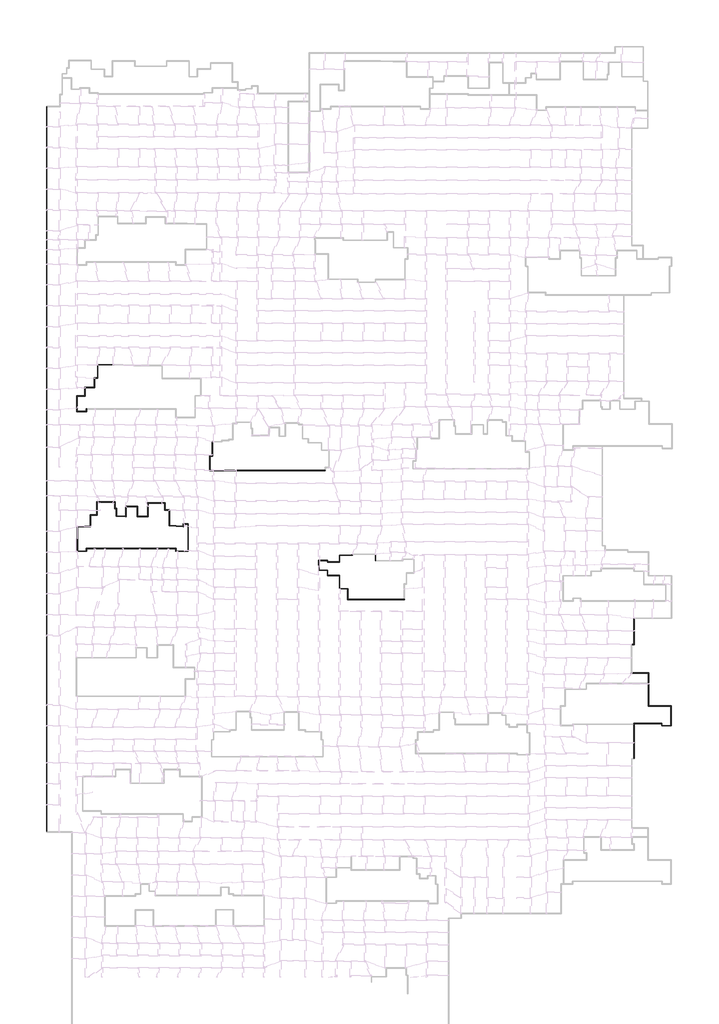
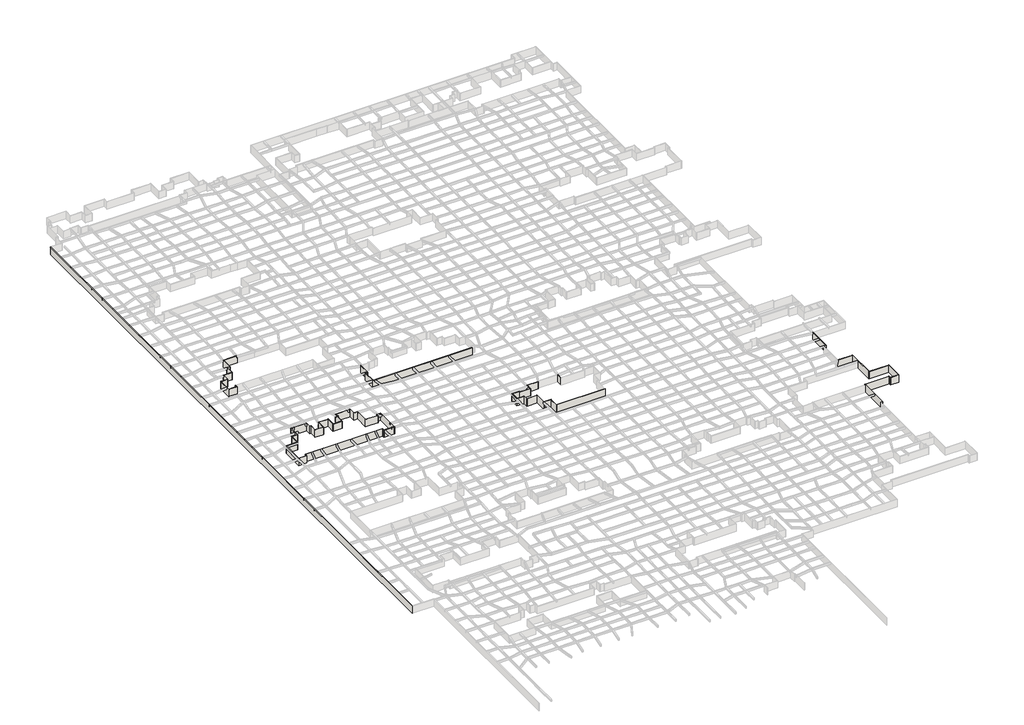
# One storey, part 5 of 45: 68 walls.
"""IFC4 building model written with IfcOpenShell, lengths in millimetres."""

from ifc_helpers import new_model, si_unit, origin, origin_with_axes, place, context, project, spatial, polyline, outline, extrude, faceted_brep, element, save

model = new_model("IFC4")

# Units and contexts
model_context = context("Model", 3, world=origin())
ifc_project = project(units=[si_unit("LENGTHUNIT", "METRE", prefix="MILLI")], contexts=[model_context])

# Site, building, storey
site = spatial("IfcSite", under=ifc_project)
building = spatial("IfcBuilding", under=site)
storey = spatial("IfcBuildingStorey", under=building, Name="户型图", Elevation=0.0)

# Walls
placement = place(None, origin())
element("IfcWall", 1, ObjectType="所有墙体", at=placement, inside=storey, context=model_context, shape_type="Brep", body=[
    faceted_brep([(-155100.5216564, 191211.9876735, 0.0), (-155100.5216564, -79588.0123265, 0.0), (-155100.5216564, -79588.0123265, 3300.0), (-155100.5216564, 191211.9876735, 3300.0), (-154980.5216564, 191211.9876735, 0.0), (-154980.5216564, 191211.9876735, 3300.0), (-154980.5216564, -79468.0123265, 3300.0), (-154980.5216564, -79588.0123265, 3300.0), (-154980.5216564, -79588.0123265, 0.0), (-154980.5216564, -79468.0123265, 0.0)], [[[0, 1, 2, 3]], [[4, 5, 6, 7, 8, 9]], [[1, 0, 4, 9, 8]], [[3, 2, 7, 6, 5]], [[0, 3, 5, 4]], [[2, 1, 8, 7]]]),
])
element("IfcWall", 2, ObjectType="所有墙体", at=placement, inside=storey, context=model_context, shape_type="Brep", body=[
    faceted_brep([(64319.4783436, -52068.0123265, 0.0), (64319.4783436, -38988.0123265, 0.0), (64319.4783436, -38868.0123265, 0.0), (64319.4783436, -38868.0123265, 3300.0), (64319.4783436, -38988.0123265, 3300.0), (64319.4783436, -52068.0123265, 3300.0), (64199.4783436, -52068.0123265, 0.0), (64199.4783436, -52068.0123265, 3300.0), (64199.4783436, -39338.8304418, 3300.0), (64199.4783436, -39218.8304418, 3300.0), (64199.4783436, -38868.0123265, 3300.0), (64199.4783436, -38868.0123265, 0.0), (64199.4783436, -39218.8304418, 0.0), (64199.4783436, -39338.8304418, 0.0)], [[[0, 1, 2, 3, 4, 5]], [[6, 7, 8, 9, 10, 11, 12, 13]], [[2, 1, 0, 6, 13, 12, 11]], [[5, 4, 3, 10, 9, 8, 7]], [[0, 5, 7, 6]], [[3, 2, 11, 10]]]),
])
element("IfcWall", 3, ObjectType="所有墙体", at=placement, inside=storey, context=model_context, shape_type="Brep", body=[
    faceted_brep([(64319.4783436, -38988.0123265, 0.0), (74599.4783436, -38988.0123265, 0.0), (74719.4783436, -38988.0123265, 0.0), (74719.4783436, -38988.0123265, 3300.0), (74599.4783436, -38988.0123265, 3300.0), (64319.4783436, -38988.0123265, 3300.0), (64319.4783436, -38868.0123265, 0.0), (64319.4783436, -38868.0123265, 3300.0), (74719.4783436, -38868.0123265, 3300.0), (74719.4783436, -38868.0123265, 0.0)], [[[0, 1, 2, 3, 4, 5]], [[6, 7, 8, 9]], [[2, 1, 0, 6, 9]], [[5, 4, 3, 8, 7]], [[0, 5, 7, 6]], [[3, 2, 9, 8]]]),
])
element("IfcWall", 4, ObjectType="所有墙体", at=placement, inside=storey, context=model_context, shape_type="Brep", body=[
    faceted_brep([(74599.4783436, -38988.0123265, 0.0), (74599.4783436, -39888.0123265, 0.0), (74599.4783436, -39888.0123265, 3300.0), (74599.4783436, -38988.0123265, 3300.0), (74719.4783436, -38988.0123265, 0.0), (74719.4783436, -38988.0123265, 3300.0), (74719.4783436, -39768.0123265, 3300.0), (74719.4783436, -39888.0123265, 3300.0), (74719.4783436, -39888.0123265, 0.0), (74719.4783436, -39768.0123265, 0.0)], [[[0, 1, 2, 3]], [[4, 5, 6, 7, 8, 9]], [[1, 0, 4, 9, 8]], [[3, 2, 7, 6, 5]], [[0, 3, 5, 4]], [[2, 1, 8, 7]]]),
])
element("IfcWall", 5, ObjectType="所有墙体", at=placement, inside=storey, context=model_context, shape_type="Brep", body=[
    faceted_brep([(74719.4783436, -39888.0123265, 0.0), (78219.4783436, -39888.0123265, 0.0), (78219.4783436, -39888.0123265, 3300.0), (74719.4783436, -39888.0123265, 3300.0), (74719.4783436, -39768.0123265, 0.0), (74719.4783436, -39768.0123265, 3300.0), (78099.4783436, -39768.0123265, 3300.0), (78219.4783436, -39768.0123265, 3300.0), (78219.4783436, -39768.0123265, 0.0), (78099.4783436, -39768.0123265, 0.0)], [[[0, 1, 2, 3]], [[4, 5, 6, 7, 8, 9]], [[1, 0, 4, 9, 8]], [[3, 2, 7, 6, 5]], [[0, 3, 5, 4]], [[2, 1, 8, 7]]]),
])
element("IfcWall", 6, ObjectType="所有墙体", at=placement, inside=storey, context=model_context, shape_type="Brep", body=[
    faceted_brep([(78219.4783436, -39768.0123265, 0.0), (78219.4783436, -32368.0123265, 0.0), (78219.4783436, -32368.0123265, 3300.0), (78219.4783436, -39768.0123265, 3300.0), (78099.4783436, -39768.0123265, 0.0), (78099.4783436, -39768.0123265, 3300.0), (78099.4783436, -32488.0123265, 3300.0), (78099.4783436, -32368.0123265, 3300.0), (78099.4783436, -32368.0123265, 0.0), (78099.4783436, -32488.0123265, 0.0)], [[[0, 1, 2, 3]], [[4, 5, 6, 7, 8, 9]], [[1, 0, 4, 9, 8]], [[3, 2, 7, 6, 5]], [[0, 3, 5, 4]], [[2, 1, 8, 7]]]),
])
element("IfcWall", 7, ObjectType="所有墙体", at=placement, inside=storey, context=model_context, shape_type="Brep", body=[
    faceted_brep([(78099.4783436, -32368.0123265, 0.0), (69819.4783436, -32368.0123265, 0.0), (69699.4783436, -32368.0123265, 0.0), (69699.4783436, -32368.0123265, 3300.0), (69819.4783436, -32368.0123265, 3300.0), (78099.4783436, -32368.0123265, 3300.0), (78099.4783436, -32488.0123265, 0.0), (78099.4783436, -32488.0123265, 3300.0), (69699.4783436, -32488.0123265, 3300.0), (69699.4783436, -32488.0123265, 0.0)], [[[0, 1, 2, 3, 4, 5]], [[6, 7, 8, 9]], [[2, 1, 0, 6, 9]], [[5, 4, 3, 8, 7]], [[0, 5, 7, 6]], [[3, 2, 9, 8]]]),
])
element("IfcWall", 8, ObjectType="所有墙体", at=placement, inside=storey, context=model_context, shape_type="Brep", body=[
    faceted_brep([(69819.4783436, -32368.0123265, 0.0), (69819.4783436, -20068.0123265, 0.0), (69819.4783436, -20068.0123265, 3300.0), (69819.4783436, -32368.0123265, 3300.0), (69699.4783436, -32368.0123265, 0.0), (69699.4783436, -32368.0123265, 3300.0), (69699.4783436, -24130.6851163, 3300.0), (69699.4783436, -24010.6851163, 3300.0), (69699.4783436, -20188.0123265, 3300.0), (69699.4783436, -20068.0123265, 3300.0), (69699.4783436, -20068.0123265, 0.0), (69699.4783436, -20188.0123265, 0.0), (69699.4783436, -24010.6851163, 0.0), (69699.4783436, -24130.6851163, 0.0)], [[[0, 1, 2, 3]], [[4, 5, 6, 7, 8, 9, 10, 11, 12, 13]], [[1, 0, 4, 13, 12, 11, 10]], [[3, 2, 9, 8, 7, 6, 5]], [[0, 3, 5, 4]], [[2, 1, 10, 9]]]),
])
element("IfcWall", 9, ObjectType="所有墙体", at=placement, inside=storey, context=model_context, shape_type="Brep", body=[
    faceted_brep([(69699.4783436, -20068.0123265, 0.0), (63419.4783436, -20068.0123265, 0.0), (63299.4783436, -20068.0123265, 0.0), (63299.4783436, -20068.0123265, 3300.0), (63419.4783436, -20068.0123265, 3300.0), (69699.4783436, -20068.0123265, 3300.0), (69699.4783436, -20188.0123265, 0.0), (69699.4783436, -20188.0123265, 3300.0), (63299.4783436, -20188.0123265, 3300.0), (63299.4783436, -20188.0123265, 0.0)], [[[0, 1, 2, 3, 4, 5]], [[6, 7, 8, 9]], [[2, 1, 0, 6, 9]], [[5, 4, 3, 8, 7]], [[0, 5, 7, 6]], [[3, 2, 9, 8]]]),
])
element("IfcWall", 10, ObjectType="所有墙体", at=placement, inside=storey, context=model_context, shape_type="Brep", body=[
    faceted_brep([(63419.4783436, -9588.0123265, 0.0), (64419.4783436, -9588.0123265, 0.0), (64419.4783436, -9588.0123265, 3300.0), (63419.4783436, -9588.0123265, 3300.0), (63419.4783436, -9468.0123265, 0.0), (63419.4783436, -9468.0123265, 3300.0), (64299.4783436, -9468.0123265, 3300.0), (64419.4783436, -9468.0123265, 3300.0), (64419.4783436, -9468.0123265, 0.0), (64299.4783436, -9468.0123265, 0.0)], [[[0, 1, 2, 3]], [[4, 5, 6, 7, 8, 9]], [[1, 0, 4, 9, 8]], [[3, 2, 7, 6, 5]], [[0, 3, 5, 4]], [[2, 1, 8, 7]]]),
])
element("IfcWall", 11, ObjectType="所有墙体", at=placement, inside=storey, context=model_context, shape_type="Brep", body=[
    faceted_brep([(64419.4783436, -9468.0123265, 0.0), (64419.4783436, 211.9876735, 0.0), (64419.4783436, 331.9876735, 0.0), (64419.4783436, 331.9876735, 3300.0), (64419.4783436, 211.9876735, 3300.0), (64419.4783436, -9468.0123265, 3300.0), (64299.4783436, -9468.0123265, 0.0), (64299.4783436, -9468.0123265, 3300.0), (64299.4783436, 331.9876735, 3300.0), (64299.4783436, 331.9876735, 0.0)], [[[0, 1, 2, 3, 4, 5]], [[6, 7, 8, 9]], [[2, 1, 0, 6, 9]], [[5, 4, 3, 8, 7]], [[0, 5, 7, 6]], [[3, 2, 9, 8]]]),
])
element("IfcWall", 12, ObjectType="所有墙体", at=placement, inside=storey, context=model_context, shape_type="Brep", body=[
    faceted_brep([(-136051.3875586, 94934.6670053, 0.0), (-136051.3875586, 90014.2865852, 0.0), (-136051.3875586, 89894.2865852, 0.0), (-136051.3875586, 89894.2865852, 3300.0), (-136051.3875586, 90014.2865852, 3300.0), (-136051.3875586, 94934.6670053, 3300.0), (-135931.3875586, 94934.6670053, 0.0), (-135931.3875586, 94934.6670053, 3300.0), (-135931.3875586, 94814.6670053, 3300.0), (-135931.3875586, 89894.2865852, 3300.0), (-135931.3875586, 89894.2865852, 0.0), (-135931.3875586, 94814.6670053, 0.0)], [[[0, 1, 2, 3, 4, 5]], [[6, 7, 8, 9, 10, 11]], [[2, 1, 0, 6, 11, 10]], [[5, 4, 3, 9, 8, 7]], [[3, 2, 10, 9]], [[0, 5, 7, 6]]]),
])
element("IfcWall", 13, ObjectType="所有墙体", at=placement, inside=storey, context=model_context, shape_type="Brep", body=[
    faceted_brep([(-136051.3875586, 90014.2865852, 0.0), (-137251.3875586, 90014.2865852, 0.0), (-137251.3875586, 90014.2865852, 3300.0), (-136051.3875586, 90014.2865852, 3300.0), (-136051.3875586, 89894.2865852, 0.0), (-136051.3875586, 89894.2865852, 3300.0), (-137131.3875586, 89894.2865852, 3300.0), (-137251.3875586, 89894.2865852, 3300.0), (-137251.3875586, 89894.2865852, 0.0), (-137131.3875586, 89894.2865852, 0.0)], [[[0, 1, 2, 3]], [[4, 5, 6, 7, 8, 9]], [[1, 0, 4, 9, 8]], [[3, 2, 7, 6, 5]], [[0, 3, 5, 4]], [[2, 1, 8, 7]]]),
])
element("IfcWall", 14, ObjectType="所有墙体", at=placement, inside=storey, context=model_context, shape_type="Brep", body=[
    faceted_brep([(-137251.3875586, 89894.2865852, 0.0), (-137251.3875586, 86414.2865852, 0.0), (-137251.3875586, 86294.2865852, 0.0), (-137251.3875586, 86294.2865852, 3300.0), (-137251.3875586, 86414.2865852, 3300.0), (-137251.3875586, 89894.2865852, 3300.0), (-137131.3875586, 89894.2865852, 0.0), (-137131.3875586, 89894.2865852, 3300.0), (-137131.3875586, 86294.2865852, 3300.0), (-137131.3875586, 86294.2865852, 0.0)], [[[0, 1, 2, 3, 4, 5]], [[6, 7, 8, 9]], [[2, 1, 0, 6, 9]], [[5, 4, 3, 8, 7]], [[0, 5, 7, 6]], [[3, 2, 9, 8]]]),
])
element("IfcWall", 15, ObjectType="所有墙体", at=placement, inside=storey, context=model_context, shape_type="Brep", body=[
    faceted_brep([(-137251.3875586, 86414.2865852, 0.0), (-140851.3875586, 86414.2865852, 0.0), (-140851.3875586, 86414.2865852, 3300.0), (-137251.3875586, 86414.2865852, 3300.0), (-137251.3875586, 86294.2865852, 0.0), (-137251.3875586, 86294.2865852, 3300.0), (-140731.3875586, 86294.2865852, 3300.0), (-140851.3875586, 86294.2865852, 3300.0), (-140851.3875586, 86294.2865852, 0.0), (-140731.3875586, 86294.2865852, 0.0)], [[[0, 1, 2, 3]], [[4, 5, 6, 7, 8, 9]], [[1, 0, 4, 9, 8]], [[3, 2, 7, 6, 5]], [[0, 3, 5, 4]], [[2, 1, 8, 7]]]),
])
element("IfcWall", 16, ObjectType="所有墙体", at=placement, inside=storey, context=model_context, shape_type="Brep", body=[
    faceted_brep([(-140851.3875586, 86294.2865852, 0.0), (-140851.3875586, 83314.2865852, 0.0), (-140851.3875586, 83194.2865852, 0.0), (-140851.3875586, 83194.2865852, 3300.0), (-140851.3875586, 83314.2865852, 3300.0), (-140851.3875586, 86294.2865852, 3300.0), (-140731.3875586, 86294.2865852, 0.0), (-140731.3875586, 86294.2865852, 3300.0), (-140731.3875586, 83194.2865852, 3300.0), (-140731.3875586, 83194.2865852, 0.0)], [[[0, 1, 2, 3, 4, 5]], [[6, 7, 8, 9]], [[2, 1, 0, 6, 9]], [[5, 4, 3, 8, 7]], [[0, 5, 7, 6]], [[3, 2, 9, 8]]]),
])
element("IfcWall", 17, ObjectType="所有墙体", at=placement, inside=storey, context=model_context, shape_type="Brep", body=[
    faceted_brep([(-140851.3875586, 83314.2865852, 0.0), (-143751.3875586, 83314.2865852, 0.0), (-143751.3875586, 83314.2865852, 3300.0), (-140851.3875586, 83314.2865852, 3300.0), (-140851.3875586, 83194.2865852, 0.0), (-140851.3875586, 83194.2865852, 3300.0), (-143631.3875586, 83194.2865852, 3300.0), (-143751.3875586, 83194.2865852, 3300.0), (-143751.3875586, 83194.2865852, 0.0), (-143631.3875586, 83194.2865852, 0.0)], [[[0, 1, 2, 3]], [[4, 5, 6, 7, 8, 9]], [[1, 0, 4, 9, 8]], [[3, 2, 7, 6, 5]], [[0, 3, 5, 4]], [[2, 1, 8, 7]]]),
])
element("IfcWall", 18, ObjectType="所有墙体", at=placement, inside=storey, context=model_context, shape_type="Brep", body=[
    faceted_brep([(-143751.3875586, 83194.2865852, 0.0), (-143751.3875586, 77394.2865852, 0.0), (-143751.3875586, 77394.2865852, 3300.0), (-143751.3875586, 83194.2865852, 3300.0), (-143631.3875586, 83194.2865852, 0.0), (-143631.3875586, 83194.2865852, 3300.0), (-143631.3875586, 77514.2865852, 3300.0), (-143631.3875586, 77394.2865852, 3300.0), (-143631.3875586, 77394.2865852, 0.0), (-143631.3875586, 77514.2865852, 0.0)], [[[0, 1, 2, 3]], [[4, 5, 6, 7, 8, 9]], [[1, 0, 4, 9, 8]], [[3, 2, 7, 6, 5]], [[0, 3, 5, 4]], [[2, 1, 8, 7]]]),
])
element("IfcWall", 19, ObjectType="所有墙体", at=placement, inside=storey, context=model_context, shape_type="Brep", body=[
    faceted_brep([(-143631.3875586, 77394.2865852, 0.0), (-140131.3875586, 77394.2865852, 0.0), (-140131.3875586, 77394.2865852, 3300.0), (-143631.3875586, 77394.2865852, 3300.0), (-143631.3875586, 77514.2865852, 0.0), (-143631.3875586, 77514.2865852, 3300.0), (-140251.3875586, 77514.2865852, 3300.0), (-140131.3875586, 77514.2865852, 3300.0), (-140131.3875586, 77514.2865852, 0.0), (-140251.3875586, 77514.2865852, 0.0)], [[[0, 1, 2, 3]], [[4, 5, 6, 7, 8, 9]], [[1, 0, 4, 9, 8]], [[3, 2, 7, 6, 5]], [[0, 3, 5, 4]], [[2, 1, 8, 7]]]),
])
element("IfcWall", 20, ObjectType="所有墙体", at=placement, inside=storey, context=model_context, shape_type="Brep", body=[
    faceted_brep([(-140131.3875586, 77514.2865852, 0.0), (-140131.3875586, 78294.2865852, 0.0), (-140131.3875586, 78414.2865852, 0.0), (-140131.3875586, 78414.2865852, 3300.0), (-140131.3875586, 78294.2865852, 3300.0), (-140131.3875586, 77514.2865852, 3300.0), (-140251.3875586, 77514.2865852, 0.0), (-140251.3875586, 77514.2865852, 3300.0), (-140251.3875586, 78414.2865852, 3300.0), (-140251.3875586, 78414.2865852, 0.0)], [[[0, 1, 2, 3, 4, 5]], [[6, 7, 8, 9]], [[2, 1, 0, 6, 9]], [[5, 4, 3, 8, 7]], [[0, 5, 7, 6]], [[3, 2, 9, 8]]]),
])
element("IfcWall", 21, ObjectType="所有墙体", at=placement, inside=storey, context=model_context, shape_type="SweptSolid", body=[
    extrude(outline(polyline([(-135931.3875586, 94934.6670053), (-129985.7714573, 94934.6670053), (-129987.8660651, 94814.6670053), (-135931.3875586, 94814.6670053), (-135931.3875586, 94934.6670053)])), origin_with_axes(), (0.0, 0.0, 1.0), 3300.0),
])
element("IfcWall", 22, ObjectType="所有墙体", at=placement, inside=storey, context=model_context, shape_type="Brep", body=[
    faceted_brep([(-51113.897353, 55455.9851813, 0.0), (-93993.897353, 55455.9851813, 0.0), (-94113.897353, 55455.9851813, 0.0), (-94113.897353, 55455.9851813, 3300.0), (-93993.897353, 55455.9851813, 3300.0), (-51113.897353, 55455.9851813, 3300.0), (-51113.897353, 55335.9851813, 0.0), (-51113.897353, 55335.9851813, 3300.0), (-94113.897353, 55335.9851813, 3300.0), (-94113.897353, 55335.9851813, 0.0)], [[[0, 1, 2, 3, 4, 5]], [[6, 7, 8, 9]], [[2, 1, 0, 6, 9]], [[5, 4, 3, 8, 7]], [[0, 5, 7, 6]], [[3, 2, 9, 8]]]),
])
element("IfcWall", 23, ObjectType="所有墙体", at=placement, inside=storey, context=model_context, shape_type="Brep", body=[
    faceted_brep([(-93993.897353, 55455.9851813, 0.0), (-93993.897353, 60835.9851813, 0.0), (-93993.897353, 60955.9851813, 0.0), (-93993.897353, 60955.9851813, 3300.0), (-93993.897353, 60835.9851813, 3300.0), (-93993.897353, 55455.9851813, 3300.0), (-94113.897353, 55455.9851813, 0.0), (-94113.897353, 55455.9851813, 3300.0), (-94113.897353, 60955.9851813, 3300.0), (-94113.897353, 60955.9851813, 0.0)], [[[0, 1, 2, 3, 4, 5]], [[6, 7, 8, 9]], [[2, 1, 0, 6, 9]], [[5, 4, 3, 8, 7]], [[0, 5, 7, 6]], [[3, 2, 9, 8]]]),
])
element("IfcWall", 24, ObjectType="所有墙体", at=placement, inside=storey, context=model_context, shape_type="Brep", body=[
    faceted_brep([(-93993.897353, 60835.9851813, 0.0), (-93093.897353, 60835.9851813, 0.0), (-93093.897353, 60835.9851813, 3300.0), (-93993.897353, 60835.9851813, 3300.0), (-93993.897353, 60955.9851813, 0.0), (-93993.897353, 60955.9851813, 3300.0), (-93213.897353, 60955.9851813, 3300.0), (-93093.897353, 60955.9851813, 3300.0), (-93093.897353, 60955.9851813, 0.0), (-93213.897353, 60955.9851813, 0.0)], [[[0, 1, 2, 3]], [[4, 5, 6, 7, 8, 9]], [[1, 0, 4, 9, 8]], [[3, 2, 7, 6, 5]], [[0, 3, 5, 4]], [[2, 1, 8, 7]]]),
])
element("IfcWall", 25, ObjectType="所有墙体", at=placement, inside=storey, context=model_context, shape_type="Brep", body=[
    faceted_brep([(-93093.897353, 60955.9851813, 0.0), (-93093.897353, 66089.1206587, 0.0), (-93093.897353, 66209.1206587, 0.0), (-93093.897353, 66209.1206587, 3300.0), (-93093.897353, 66089.1206587, 3300.0), (-93093.897353, 60955.9851813, 3300.0), (-93213.897353, 60955.9851813, 0.0), (-93213.897353, 60955.9851813, 3300.0), (-93213.897353, 66209.1206587, 3300.0), (-93213.897353, 66209.1206587, 0.0)], [[[0, 1, 2, 3, 4, 5]], [[6, 7, 8, 9]], [[2, 1, 0, 6, 9]], [[5, 4, 3, 8, 7]], [[0, 5, 7, 6]], [[3, 2, 9, 8]]]),
])
element("IfcWall", 26, ObjectType="所有墙体", at=placement, inside=storey, context=model_context, shape_type="Brep", body=[
    faceted_brep([(-138710.8272977, 38758.3043214, 0.0), (-138710.8272977, 34629.9375221, 0.0), (-138710.8272977, 34509.9375221, 0.0), (-138710.8272977, 34509.9375221, 3300.0), (-138710.8272977, 34629.9375221, 3300.0), (-138710.8272977, 38758.3043214, 3300.0), (-138590.8272977, 38758.3043214, 0.0), (-138590.8272977, 38758.3043214, 3300.0), (-138590.8272977, 34509.9375221, 3300.0), (-138590.8272977, 34509.9375221, 0.0)], [[[0, 1, 2, 3, 4, 5]], [[6, 7, 8, 9]], [[2, 1, 0, 6, 9]], [[5, 4, 3, 8, 7]], [[3, 2, 9, 8]], [[0, 5, 7, 6]]]),
])
element("IfcWall", 27, ObjectType="所有墙体", at=placement, inside=storey, context=model_context, shape_type="Brep", body=[
    faceted_brep([(-138710.8272977, 34629.9375221, 0.0), (-143610.8272977, 34629.9375221, 0.0), (-143610.8272977, 34629.9375221, 3300.0), (-138710.8272977, 34629.9375221, 3300.0), (-138710.8272977, 34509.9375221, 0.0), (-138710.8272977, 34509.9375221, 3300.0), (-143490.8272977, 34509.9375221, 3300.0), (-143610.8272977, 34509.9375221, 3300.0), (-143610.8272977, 34509.9375221, 0.0), (-143490.8272977, 34509.9375221, 0.0)], [[[0, 1, 2, 3]], [[4, 5, 6, 7, 8, 9]], [[1, 0, 4, 9, 8]], [[3, 2, 7, 6, 5]], [[0, 3, 5, 4]], [[2, 1, 8, 7]]]),
])
element("IfcWall", 28, ObjectType="所有墙体", at=placement, inside=storey, context=model_context, shape_type="Brep", body=[
    faceted_brep([(-143610.8272977, 34509.9375221, 0.0), (-143610.8272977, 25209.9375221, 0.0), (-143610.8272977, 25209.9375221, 3300.0), (-143610.8272977, 34509.9375221, 3300.0), (-143490.8272977, 34509.9375221, 0.0), (-143490.8272977, 34509.9375221, 3300.0), (-143490.8272977, 25329.9375221, 3300.0), (-143490.8272977, 25209.9375221, 3300.0), (-143490.8272977, 25209.9375221, 0.0), (-143490.8272977, 25329.9375221, 0.0)], [[[0, 1, 2, 3]], [[4, 5, 6, 7, 8, 9]], [[1, 0, 4, 9, 8]], [[3, 2, 7, 6, 5]], [[0, 3, 5, 4]], [[2, 1, 8, 7]]]),
])
element("IfcWall", 29, ObjectType="所有墙体", at=placement, inside=storey, context=model_context, shape_type="Brep", body=[
    faceted_brep([(-143490.8272977, 25209.9375221, 0.0), (-140090.8272977, 25209.9375221, 0.0), (-140090.8272977, 25209.9375221, 3300.0), (-143490.8272977, 25209.9375221, 3300.0), (-143490.8272977, 25329.9375221, 0.0), (-143490.8272977, 25329.9375221, 3300.0), (-140210.8272977, 25329.9375221, 3300.0), (-140090.8272977, 25329.9375221, 3300.0), (-140090.8272977, 25329.9375221, 0.0), (-140210.8272977, 25329.9375221, 0.0)], [[[0, 1, 2, 3]], [[4, 5, 6, 7, 8, 9]], [[1, 0, 4, 9, 8]], [[3, 2, 7, 6, 5]], [[0, 3, 5, 4]], [[2, 1, 8, 7]]]),
])
element("IfcWall", 30, ObjectType="所有墙体", at=placement, inside=storey, context=model_context, shape_type="Brep", body=[
    faceted_brep([(-140090.8272977, 25329.9375221, 0.0), (-140090.8272977, 26209.9375221, 0.0), (-140090.8272977, 26329.9375221, 0.0), (-140090.8272977, 26329.9375221, 3300.0), (-140090.8272977, 26209.9375221, 3300.0), (-140090.8272977, 25329.9375221, 3300.0), (-140210.8272977, 25329.9375221, 0.0), (-140210.8272977, 25329.9375221, 3300.0), (-140210.8272977, 26329.9375221, 3300.0), (-140210.8272977, 26329.9375221, 0.0)], [[[0, 1, 2, 3, 4, 5]], [[6, 7, 8, 9]], [[2, 1, 0, 6, 9]], [[5, 4, 3, 8, 7]], [[0, 5, 7, 6]], [[3, 2, 9, 8]]]),
])
element("IfcWall", 31, ObjectType="所有墙体", at=placement, inside=storey, context=model_context, shape_type="Brep", body=[
    faceted_brep([(-140090.8272977, 26209.9375221, 0.0), (-106810.8272977, 26209.9375221, 0.0), (-106690.8272977, 26209.9375221, 0.0), (-106690.8272977, 26209.9375221, 3300.0), (-106810.8272977, 26209.9375221, 3300.0), (-140090.8272977, 26209.9375221, 3300.0), (-140090.8272977, 26329.9375221, 0.0), (-140090.8272977, 26329.9375221, 3300.0), (-106690.8272977, 26329.9375221, 3300.0), (-106690.8272977, 26329.9375221, 0.0)], [[[0, 1, 2, 3, 4, 5]], [[6, 7, 8, 9]], [[2, 1, 0, 6, 9]], [[5, 4, 3, 8, 7]], [[0, 5, 7, 6]], [[3, 2, 9, 8]]]),
])
element("IfcWall", 32, ObjectType="所有墙体", at=placement, inside=storey, context=model_context, shape_type="Brep", body=[
    faceted_brep([(-106810.8272977, 26209.9375221, 0.0), (-106810.8272977, 25209.9375221, 0.0), (-106810.8272977, 25209.9375221, 3300.0), (-106810.8272977, 26209.9375221, 3300.0), (-106690.8272977, 26209.9375221, 0.0), (-106690.8272977, 26209.9375221, 3300.0), (-106690.8272977, 25329.9375221, 3300.0), (-106690.8272977, 25209.9375221, 3300.0), (-106690.8272977, 25209.9375221, 0.0), (-106690.8272977, 25329.9375221, 0.0)], [[[0, 1, 2, 3]], [[4, 5, 6, 7, 8, 9]], [[1, 0, 4, 9, 8]], [[3, 2, 7, 6, 5]], [[0, 3, 5, 4]], [[2, 1, 8, 7]]]),
])
element("IfcWall", 33, ObjectType="所有墙体", at=placement, inside=storey, context=model_context, shape_type="Brep", body=[
    faceted_brep([(-106690.8272977, 25209.9375221, 0.0), (-102190.8272977, 25209.9375221, 0.0), (-102190.8272977, 25209.9375221, 3300.0), (-106690.8272977, 25209.9375221, 3300.0), (-106690.8272977, 25329.9375221, 0.0), (-106690.8272977, 25329.9375221, 3300.0), (-102310.8272977, 25329.9375221, 3300.0), (-102190.8272977, 25329.9375221, 3300.0), (-102190.8272977, 25329.9375221, 0.0), (-102310.8272977, 25329.9375221, 0.0)], [[[0, 1, 2, 3]], [[4, 5, 6, 7, 8, 9]], [[1, 0, 4, 9, 8]], [[3, 2, 7, 6, 5]], [[0, 3, 5, 4]], [[2, 1, 8, 7]]]),
])
element("IfcWall", 34, ObjectType="所有墙体", at=placement, inside=storey, context=model_context, shape_type="Brep", body=[
    faceted_brep([(-102190.8272977, 25329.9375221, 0.0), (-102190.8272977, 35529.9375221, 0.0), (-102190.8272977, 35529.9375221, 3300.0), (-102190.8272977, 25329.9375221, 3300.0), (-102310.8272977, 25329.9375221, 0.0), (-102310.8272977, 25329.9375221, 3300.0), (-102310.8272977, 35409.9375221, 3300.0), (-102310.8272977, 35529.9375221, 3300.0), (-102310.8272977, 35529.9375221, 0.0), (-102310.8272977, 35409.9375221, 0.0)], [[[0, 1, 2, 3]], [[4, 5, 6, 7, 8, 9]], [[1, 0, 4, 9, 8]], [[3, 2, 7, 6, 5]], [[0, 3, 5, 4]], [[2, 1, 8, 7]]]),
])
element("IfcWall", 35, ObjectType="所有墙体", at=placement, inside=storey, context=model_context, shape_type="Brep", body=[
    faceted_brep([(-102310.8272977, 35529.9375221, 0.0), (-104010.8272977, 35529.9375221, 0.0), (-104010.8272977, 35529.9375221, 3300.0), (-102310.8272977, 35529.9375221, 3300.0), (-102310.8272977, 35409.9375221, 0.0), (-102310.8272977, 35409.9375221, 3300.0), (-103890.8272977, 35409.9375221, 3300.0), (-104010.8272977, 35409.9375221, 3300.0), (-104010.8272977, 35409.9375221, 0.0), (-103890.8272977, 35409.9375221, 0.0)], [[[0, 1, 2, 3]], [[4, 5, 6, 7, 8, 9]], [[1, 0, 4, 9, 8]], [[3, 2, 7, 6, 5]], [[0, 3, 5, 4]], [[2, 1, 8, 7]]]),
])
element("IfcWall", 36, ObjectType="所有墙体", at=placement, inside=storey, context=model_context, shape_type="Brep", body=[
    faceted_brep([(-104010.8272977, 35409.9375221, 0.0), (-104010.8272977, 34633.1643296, 0.0), (-104010.8272977, 34512.9996481, 0.0), (-104010.8272977, 34512.9996481, 3300.0), (-104010.8272977, 34633.1643296, 3300.0), (-104010.8272977, 35409.9375221, 3300.0), (-103890.8272977, 35409.9375221, 0.0), (-103890.8272977, 35409.9375221, 3300.0), (-103890.8272977, 34506.7107146, 3300.0), (-103890.8272977, 34506.7107146, 0.0)], [[[0, 1, 2, 3, 4, 5]], [[6, 7, 8, 9]], [[2, 1, 0, 6, 9]], [[5, 4, 3, 8, 7]], [[0, 5, 7, 6]], [[3, 2, 9, 8]]]),
])
element("IfcWall", 37, ObjectType="所有墙体", at=placement, inside=storey, context=model_context, shape_type="Brep", body=[
    faceted_brep([(-104010.8272977, 34633.1643296, 0.0), (-109183.5638319, 34904.2559642, 0.0), (-109303.5638319, 34910.5448977, 0.0), (-109303.5638319, 34910.5448977, 3300.0), (-109183.5638319, 34904.2559642, 3300.0), (-104010.8272977, 34633.1643296, 3300.0), (-104010.8272977, 34512.9996481, 0.0), (-104010.8272977, 34512.9996481, 3300.0), (-109303.5638319, 34790.3802162, 3300.0), (-109303.5638319, 34790.3802162, 0.0)], [[[0, 1, 2, 3, 4, 5]], [[6, 7, 8, 9]], [[2, 1, 0, 6, 9]], [[5, 4, 3, 8, 7]], [[0, 5, 7, 6]], [[3, 2, 9, 8]]]),
])
element("IfcWall", 38, ObjectType="所有墙体", at=placement, inside=storey, context=model_context, shape_type="Brep", body=[
    faceted_brep([(-109183.5638319, 34904.2559642, 0.0), (-109183.5638319, 40707.3180902, 0.0), (-109183.5638319, 40707.3180902, 3300.0), (-109183.5638319, 34904.2559642, 3300.0), (-109303.5638319, 34910.5448977, 0.0), (-109303.5638319, 34910.5448977, 3300.0), (-109303.5638319, 40587.3180902, 3300.0), (-109303.5638319, 40707.3180902, 3300.0), (-109303.5638319, 40707.3180902, 0.0), (-109303.5638319, 40587.3180902, 0.0)], [[[0, 1, 2, 3]], [[4, 5, 6, 7, 8, 9]], [[1, 0, 4, 9, 8]], [[3, 2, 7, 6, 5]], [[0, 3, 5, 4]], [[2, 1, 8, 7]]]),
])
element("IfcWall", 39, ObjectType="所有墙体", at=placement, inside=storey, context=model_context, shape_type="Brep", body=[
    faceted_brep([(-109303.5638319, 40707.3180902, 0.0), (-110783.5638319, 40707.3180902, 0.0), (-110903.5638319, 40707.3180902, 0.0), (-110903.5638319, 40707.3180902, 3300.0), (-110783.5638319, 40707.3180902, 3300.0), (-109303.5638319, 40707.3180902, 3300.0), (-109303.5638319, 40587.3180902, 0.0), (-109303.5638319, 40587.3180902, 3300.0), (-110903.5638319, 40587.3180902, 3300.0), (-110903.5638319, 40587.3180902, 0.0)], [[[0, 1, 2, 3, 4, 5]], [[6, 7, 8, 9]], [[2, 1, 0, 6, 9]], [[5, 4, 3, 8, 7]], [[0, 5, 7, 6]], [[3, 2, 9, 8]]]),
])
element("IfcWall", 40, ObjectType="所有墙体", at=placement, inside=storey, context=model_context, shape_type="Brep", body=[
    faceted_brep([(-110783.5638319, 40707.3180902, 0.0), (-110783.5638319, 43407.3180902, 0.0), (-110783.5638319, 43407.3180902, 3300.0), (-110783.5638319, 40707.3180902, 3300.0), (-110903.5638319, 40707.3180902, 0.0), (-110903.5638319, 40707.3180902, 3300.0), (-110903.5638319, 43287.3180902, 3300.0), (-110903.5638319, 43407.3180902, 3300.0), (-110903.5638319, 43407.3180902, 0.0), (-110903.5638319, 43287.3180902, 0.0)], [[[0, 1, 2, 3]], [[4, 5, 6, 7, 8, 9]], [[1, 0, 4, 9, 8]], [[3, 2, 7, 6, 5]], [[0, 3, 5, 4]], [[2, 1, 8, 7]]]),
])
element("IfcWall", 41, ObjectType="所有墙体", at=placement, inside=storey, context=model_context, shape_type="Brep", body=[
    faceted_brep([(-110903.5638319, 43407.3180902, 0.0), (-117342.3379894, 43407.3180902, 0.0), (-117342.3379894, 43407.3180902, 3300.0), (-110903.5638319, 43407.3180902, 3300.0), (-110903.5638319, 43287.3180902, 0.0), (-110903.5638319, 43287.3180902, 3300.0), (-117222.3379894, 43287.3180902, 3300.0), (-117342.3379894, 43287.3180902, 3300.0), (-117342.3379894, 43287.3180902, 0.0), (-117222.3379894, 43287.3180902, 0.0)], [[[0, 1, 2, 3]], [[4, 5, 6, 7, 8, 9]], [[1, 0, 4, 9, 8]], [[3, 2, 7, 6, 5]], [[0, 3, 5, 4]], [[2, 1, 8, 7]]]),
])
element("IfcWall", 42, ObjectType="所有墙体", at=placement, inside=storey, context=model_context, shape_type="Brep", body=[
    faceted_brep([(-117342.3379894, 43287.3180902, 0.0), (-117342.3379894, 38307.3180902, 0.0), (-117342.3379894, 38187.3180902, 0.0), (-117342.3379894, 38187.3180902, 3300.0), (-117342.3379894, 38307.3180902, 3300.0), (-117342.3379894, 43287.3180902, 3300.0), (-117222.3379894, 43287.3180902, 0.0), (-117222.3379894, 43287.3180902, 3300.0), (-117222.3379894, 38187.3180902, 3300.0), (-117222.3379894, 38187.3180902, 0.0)], [[[0, 1, 2, 3, 4, 5]], [[6, 7, 8, 9]], [[2, 1, 0, 6, 9]], [[5, 4, 3, 8, 7]], [[0, 5, 7, 6]], [[3, 2, 9, 8]]]),
])
element("IfcWall", 43, ObjectType="所有墙体", at=placement, inside=storey, context=model_context, shape_type="Brep", body=[
    faceted_brep([(-117342.3379894, 38307.3180902, 0.0), (-121122.3379894, 38307.3180902, 0.0), (-121242.3379894, 38307.3180902, 0.0), (-121242.3379894, 38307.3180902, 3300.0), (-121122.3379894, 38307.3180902, 3300.0), (-117342.3379894, 38307.3180902, 3300.0), (-117342.3379894, 38187.3180902, 0.0), (-117342.3379894, 38187.3180902, 3300.0), (-121242.3379894, 38187.3180902, 3300.0), (-121242.3379894, 38187.3180902, 0.0)], [[[0, 1, 2, 3, 4, 5]], [[6, 7, 8, 9]], [[2, 1, 0, 6, 9]], [[5, 4, 3, 8, 7]], [[0, 5, 7, 6]], [[3, 2, 9, 8]]]),
])
element("IfcWall", 44, ObjectType="所有墙体", at=placement, inside=storey, context=model_context, shape_type="Brep", body=[
    faceted_brep([(-121122.3379894, 38307.3180902, 0.0), (-121122.3379894, 42007.3180902, 0.0), (-121122.3379894, 42007.3180902, 3300.0), (-121122.3379894, 38307.3180902, 3300.0), (-121242.3379894, 38307.3180902, 0.0), (-121242.3379894, 38307.3180902, 3300.0), (-121242.3379894, 41887.3180902, 3300.0), (-121242.3379894, 42007.3180902, 3300.0), (-121242.3379894, 42007.3180902, 0.0), (-121242.3379894, 41887.3180902, 0.0)], [[[0, 1, 2, 3]], [[4, 5, 6, 7, 8, 9]], [[1, 0, 4, 9, 8]], [[3, 2, 7, 6, 5]], [[0, 3, 5, 4]], [[2, 1, 8, 7]]]),
])
element("IfcWall", 45, ObjectType="所有墙体", at=placement, inside=storey, context=model_context, shape_type="Brep", body=[
    faceted_brep([(-121242.3379894, 42007.3180902, 0.0), (-125470.2525282, 42007.3180902, 0.0), (-125470.2525282, 42007.3180902, 3300.0), (-121242.3379894, 42007.3180902, 3300.0), (-121242.3379894, 41887.3180902, 0.0), (-121242.3379894, 41887.3180902, 3300.0), (-125350.2525282, 41887.3180902, 3300.0), (-125470.2525282, 41887.3180902, 3300.0), (-125470.2525282, 41887.3180902, 0.0), (-125350.2525282, 41887.3180902, 0.0)], [[[0, 1, 2, 3]], [[4, 5, 6, 7, 8, 9]], [[1, 0, 4, 9, 8]], [[3, 2, 7, 6, 5]], [[0, 3, 5, 4]], [[2, 1, 8, 7]]]),
])
element("IfcWall", 46, ObjectType="所有墙体", at=placement, inside=storey, context=model_context, shape_type="Brep", body=[
    faceted_brep([(-125470.2525282, 41887.3180902, 0.0), (-125470.2525282, 38310.5448977, 0.0), (-125470.2525282, 38190.3802162, 0.0), (-125470.2525282, 38190.3802162, 3300.0), (-125470.2525282, 38310.5448977, 3300.0), (-125470.2525282, 41887.3180902, 3300.0), (-125350.2525282, 41887.3180902, 0.0), (-125350.2525282, 41887.3180902, 3300.0), (-125350.2525282, 38184.0912827, 3300.0), (-125350.2525282, 38184.0912827, 0.0)], [[[0, 1, 2, 3, 4, 5]], [[6, 7, 8, 9]], [[2, 1, 0, 6, 9]], [[5, 4, 3, 8, 7]], [[0, 5, 7, 6]], [[3, 2, 9, 8]]]),
])
element("IfcWall", 47, ObjectType="所有墙体", at=placement, inside=storey, context=model_context, shape_type="Brep", body=[
    faceted_brep([(-125470.2525282, 38310.5448977, 0.0), (-128945.3188533, 38492.6654067, 0.0), (-129065.3188533, 38498.9543402, 0.0), (-129065.3188533, 38498.9543402, 3300.0), (-128945.3188533, 38492.6654067, 3300.0), (-125470.2525282, 38310.5448977, 3300.0), (-125470.2525282, 38190.3802162, 0.0), (-125470.2525282, 38190.3802162, 3300.0), (-129065.3188533, 38378.7896587, 3300.0), (-129065.3188533, 38378.7896587, 0.0)], [[[0, 1, 2, 3, 4, 5]], [[6, 7, 8, 9]], [[2, 1, 0, 6, 9]], [[5, 4, 3, 8, 7]], [[0, 5, 7, 6]], [[3, 2, 9, 8]]]),
])
element("IfcWall", 48, ObjectType="所有墙体", at=placement, inside=storey, context=model_context, shape_type="Brep", body=[
    faceted_brep([(-128945.3188533, 38492.6654067, 0.0), (-128945.3188533, 41295.7275327, 0.0), (-128945.3188533, 41295.7275327, 3300.0), (-128945.3188533, 38492.6654067, 3300.0), (-129065.3188533, 38498.9543402, 0.0), (-129065.3188533, 38498.9543402, 3300.0), (-129065.3188533, 41175.7275327, 3300.0), (-129065.3188533, 41295.7275327, 3300.0), (-129065.3188533, 41295.7275327, 0.0), (-129065.3188533, 41175.7275327, 0.0)], [[[0, 1, 2, 3]], [[4, 5, 6, 7, 8, 9]], [[1, 0, 4, 9, 8]], [[3, 2, 7, 6, 5]], [[0, 3, 5, 4]], [[2, 1, 8, 7]]]),
])
element("IfcWall", 49, ObjectType="所有墙体", at=placement, inside=storey, context=model_context, shape_type="Brep", body=[
    faceted_brep([(-129065.3188533, 41295.7275327, 0.0), (-129445.3188533, 41295.7275327, 0.0), (-129565.3188533, 41295.7275327, 0.0), (-129565.3188533, 41295.7275327, 3300.0), (-129445.3188533, 41295.7275327, 3300.0), (-129065.3188533, 41295.7275327, 3300.0), (-129065.3188533, 41175.7275327, 0.0), (-129065.3188533, 41175.7275327, 3300.0), (-129565.3188533, 41175.7275327, 3300.0), (-129565.3188533, 41175.7275327, 0.0)], [[[0, 1, 2, 3, 4, 5]], [[6, 7, 8, 9]], [[2, 1, 0, 6, 9]], [[5, 4, 3, 8, 7]], [[0, 5, 7, 6]], [[3, 2, 9, 8]]]),
])
element("IfcWall", 50, ObjectType="所有墙体", at=placement, inside=storey, context=model_context, shape_type="Brep", body=[
    faceted_brep([(-129445.3188533, 41295.7275327, 0.0), (-129445.3188533, 43695.7275327, 0.0), (-129445.3188533, 43695.7275327, 3300.0), (-129445.3188533, 41295.7275327, 3300.0), (-129565.3188533, 41295.7275327, 0.0), (-129565.3188533, 41295.7275327, 3300.0), (-129565.3188533, 43575.7275327, 3300.0), (-129565.3188533, 43695.7275327, 3300.0), (-129565.3188533, 43695.7275327, 0.0), (-129565.3188533, 43575.7275327, 0.0)], [[[0, 1, 2, 3]], [[4, 5, 6, 7, 8, 9]], [[1, 0, 4, 9, 8]], [[3, 2, 7, 6, 5]], [[0, 3, 5, 4]], [[2, 1, 8, 7]]]),
])
element("IfcWall", 51, ObjectType="所有墙体", at=placement, inside=storey, context=model_context, shape_type="Brep", body=[
    faceted_brep([(-129565.3188533, 43695.7275327, 0.0), (-136365.3188533, 43695.7275327, 0.0), (-136365.3188533, 43695.7275327, 3300.0), (-129565.3188533, 43695.7275327, 3300.0), (-129565.3188533, 43575.7275327, 0.0), (-129565.3188533, 43575.7275327, 3300.0), (-136245.3188533, 43575.7275327, 3300.0), (-136365.3188533, 43575.7275327, 3300.0), (-136365.3188533, 43575.7275327, 0.0), (-136245.3188533, 43575.7275327, 0.0)], [[[0, 1, 2, 3]], [[4, 5, 6, 7, 8, 9]], [[1, 0, 4, 9, 8]], [[3, 2, 7, 6, 5]], [[0, 3, 5, 4]], [[2, 1, 8, 7]]]),
])
element("IfcWall", 52, ObjectType="所有墙体", at=placement, inside=storey, context=model_context, shape_type="Brep", body=[
    faceted_brep([(-136365.3188533, 43575.7275327, 0.0), (-136365.3188533, 38878.3043214, 0.0), (-136365.3188533, 38758.3043214, 0.0), (-136365.3188533, 38758.3043214, 3300.0), (-136365.3188533, 38878.3043214, 3300.0), (-136365.3188533, 43575.7275327, 3300.0), (-136245.3188533, 43575.7275327, 0.0), (-136245.3188533, 43575.7275327, 3300.0), (-136245.3188533, 38758.3043214, 3300.0), (-136245.3188533, 38758.3043214, 0.0)], [[[0, 1, 2, 3, 4, 5]], [[6, 7, 8, 9]], [[2, 1, 0, 6, 9]], [[5, 4, 3, 8, 7]], [[0, 5, 7, 6]], [[3, 2, 9, 8]]]),
])
element("IfcWall", 53, ObjectType="所有墙体", at=placement, inside=storey, context=model_context, shape_type="Brep", body=[
    faceted_brep([(-136365.3188533, 38878.3043214, 0.0), (-138710.8272977, 38878.3043214, 0.0), (-138710.8272977, 38878.3043214, 3300.0), (-136365.3188533, 38878.3043214, 3300.0), (-136365.3188533, 38758.3043214, 0.0), (-136365.3188533, 38758.3043214, 3300.0), (-138590.8272977, 38758.3043214, 3300.0), (-138710.8272977, 38758.3043214, 3300.0), (-138710.8272977, 38758.3043214, 0.0), (-138590.8272977, 38758.3043214, 0.0)], [[[0, 1, 2, 3]], [[4, 5, 6, 7, 8, 9]], [[1, 0, 4, 9, 8]], [[3, 2, 7, 6, 5]], [[0, 3, 5, 4]], [[2, 1, 8, 7]]]),
])
element("IfcWall", 54, ObjectType="所有墙体", at=placement, inside=storey, context=model_context, shape_type="Brep", body=[
    faceted_brep([(-40949.3626959, 24139.6283958, 0.0), (-40949.3626959, 23859.6283958, 0.0), (-40949.3626959, 23739.6283958, 0.0), (-40949.3626959, 23739.6283958, 3300.0), (-40949.3626959, 23859.6283958, 3300.0), (-40949.3626959, 24139.6283958, 3300.0), (-40829.3626959, 24139.6283958, 0.0), (-40829.3626959, 24139.6283958, 3300.0), (-40829.3626959, 23739.6283958, 3300.0), (-40829.3626959, 23739.6283958, 0.0)], [[[0, 1, 2, 3, 4, 5]], [[6, 7, 8, 9]], [[2, 1, 0, 6, 9]], [[5, 4, 3, 8, 7]], [[0, 5, 7, 6]], [[3, 2, 9, 8]]]),
])
element("IfcWall", 55, ObjectType="所有墙体", at=placement, inside=storey, context=model_context, shape_type="Brep", body=[
    faceted_brep([(-40949.3626959, 23859.6283958, 0.0), (-45731.0209029, 23859.6283958, 0.0), (-45731.0209029, 23859.6283958, 3300.0), (-40949.3626959, 23859.6283958, 3300.0), (-40949.3626959, 23739.6283958, 0.0), (-40949.3626959, 23739.6283958, 3300.0), (-45611.0209029, 23739.6283958, 3300.0), (-45731.0209029, 23739.6283958, 3300.0), (-45731.0209029, 23739.6283958, 0.0), (-45611.0209029, 23739.6283958, 0.0)], [[[0, 1, 2, 3]], [[4, 5, 6, 7, 8, 9]], [[1, 0, 4, 9, 8]], [[3, 2, 7, 6, 5]], [[0, 3, 5, 4]], [[2, 1, 8, 7]]]),
])
element("IfcWall", 56, ObjectType="所有墙体", at=placement, inside=storey, context=model_context, shape_type="Brep", body=[
    faceted_brep([(-45731.0209029, 23739.6283958, 0.0), (-45731.0209029, 21359.6283958, 0.0), (-45731.0209029, 21239.6283958, 0.0), (-45731.0209029, 21239.6283958, 3300.0), (-45731.0209029, 21359.6283958, 3300.0), (-45731.0209029, 23739.6283958, 3300.0), (-45611.0209029, 23739.6283958, 0.0), (-45611.0209029, 23739.6283958, 3300.0), (-45611.0209029, 21239.6283958, 3300.0), (-45611.0209029, 21239.6283958, 0.0)], [[[0, 1, 2, 3, 4, 5]], [[6, 7, 8, 9]], [[2, 1, 0, 6, 9]], [[5, 4, 3, 8, 7]], [[0, 5, 7, 6]], [[3, 2, 9, 8]]]),
])
element("IfcWall", 57, ObjectType="所有墙体", at=placement, inside=storey, context=model_context, shape_type="Brep", body=[
    faceted_brep([(-45731.0209029, 21359.6283958, 0.0), (-50111.0209029, 21359.6283958, 0.0), (-50231.0209029, 21359.6283958, 0.0), (-50231.0209029, 21359.6283958, 3300.0), (-50111.0209029, 21359.6283958, 3300.0), (-45731.0209029, 21359.6283958, 3300.0), (-45731.0209029, 21239.6283958, 0.0), (-45731.0209029, 21239.6283958, 3300.0), (-50231.0209029, 21239.6283958, 3300.0), (-50231.0209029, 21239.6283958, 0.0)], [[[0, 1, 2, 3, 4, 5]], [[6, 7, 8, 9]], [[2, 1, 0, 6, 9]], [[5, 4, 3, 8, 7]], [[0, 5, 7, 6]], [[3, 2, 9, 8]]]),
])
element("IfcWall", 58, ObjectType="所有墙体", at=placement, inside=storey, context=model_context, shape_type="Brep", body=[
    faceted_brep([(-50111.0209029, 21359.6283958, 0.0), (-50111.0209029, 21859.6283958, 0.0), (-50111.0209029, 21859.6283958, 3300.0), (-50111.0209029, 21359.6283958, 3300.0), (-50231.0209029, 21359.6283958, 0.0), (-50231.0209029, 21359.6283958, 3300.0), (-50231.0209029, 21739.6283958, 3300.0), (-50231.0209029, 21859.6283958, 3300.0), (-50231.0209029, 21859.6283958, 0.0), (-50231.0209029, 21739.6283958, 0.0)], [[[0, 1, 2, 3]], [[4, 5, 6, 7, 8, 9]], [[1, 0, 4, 9, 8]], [[3, 2, 7, 6, 5]], [[0, 3, 5, 4]], [[2, 1, 8, 7]]]),
])
element("IfcWall", 59, ObjectType="所有墙体", at=placement, inside=storey, context=model_context, shape_type="Brep", body=[
    faceted_brep([(-50231.0209029, 21859.6283958, 0.0), (-53431.0209029, 21859.6283958, 0.0), (-53431.0209029, 21859.6283958, 3300.0), (-50231.0209029, 21859.6283958, 3300.0), (-50231.0209029, 21739.6283958, 0.0), (-50231.0209029, 21739.6283958, 3300.0), (-53311.0209029, 21739.6283958, 3300.0), (-53431.0209029, 21739.6283958, 3300.0), (-53431.0209029, 21739.6283958, 0.0), (-53311.0209029, 21739.6283958, 0.0)], [[[0, 1, 2, 3]], [[4, 5, 6, 7, 8, 9]], [[1, 0, 4, 9, 8]], [[3, 2, 7, 6, 5]], [[0, 3, 5, 4]], [[2, 1, 8, 7]]]),
])
element("IfcWall", 60, ObjectType="所有墙体", at=placement, inside=storey, context=model_context, shape_type="Brep", body=[
    faceted_brep([(-53431.0209029, 21739.6283958, 0.0), (-53431.0209029, 18139.6283958, 0.0), (-53431.0209029, 18139.6283958, 3300.0), (-53431.0209029, 21739.6283958, 3300.0), (-53311.0209029, 21739.6283958, 0.0), (-53311.0209029, 21739.6283958, 3300.0), (-53311.0209029, 18259.6283958, 3300.0), (-53311.0209029, 18139.6283958, 3300.0), (-53311.0209029, 18139.6283958, 0.0), (-53311.0209029, 18259.6283958, 0.0)], [[[0, 1, 2, 3]], [[4, 5, 6, 7, 8, 9]], [[1, 0, 4, 9, 8]], [[3, 2, 7, 6, 5]], [[0, 3, 5, 4]], [[2, 1, 8, 7]]]),
])
element("IfcWall", 61, ObjectType="所有墙体", at=placement, inside=storey, context=model_context, shape_type="Brep", body=[
    faceted_brep([(-53311.0209029, 18139.6283958, 0.0), (-50231.0209029, 18139.6283958, 0.0), (-50111.0209029, 18139.6283958, 0.0), (-50111.0209029, 18139.6283958, 3300.0), (-50231.0209029, 18139.6283958, 3300.0), (-53311.0209029, 18139.6283958, 3300.0), (-53311.0209029, 18259.6283958, 0.0), (-53311.0209029, 18259.6283958, 3300.0), (-50111.0209029, 18259.6283958, 3300.0), (-50111.0209029, 18259.6283958, 0.0)], [[[0, 1, 2, 3, 4, 5]], [[6, 7, 8, 9]], [[2, 1, 0, 6, 9]], [[5, 4, 3, 8, 7]], [[0, 5, 7, 6]], [[3, 2, 9, 8]]]),
])
element("IfcWall", 62, ObjectType="所有墙体", at=placement, inside=storey, context=model_context, shape_type="Brep", body=[
    faceted_brep([(-50231.0209029, 18139.6283958, 0.0), (-50231.0209029, 16139.6283958, 0.0), (-50231.0209029, 16139.6283958, 3300.0), (-50231.0209029, 18139.6283958, 3300.0), (-50111.0209029, 18139.6283958, 0.0), (-50111.0209029, 18139.6283958, 3300.0), (-50111.0209029, 16259.6283958, 3300.0), (-50111.0209029, 16139.6283958, 3300.0), (-50111.0209029, 16139.6283958, 0.0), (-50111.0209029, 16259.6283958, 0.0)], [[[0, 1, 2, 3]], [[4, 5, 6, 7, 8, 9]], [[1, 0, 4, 9, 8]], [[3, 2, 7, 6, 5]], [[0, 3, 5, 4]], [[2, 1, 8, 7]]]),
])
element("IfcWall", 63, ObjectType="所有墙体", at=placement, inside=storey, context=model_context, shape_type="Brep", body=[
    faceted_brep([(-50111.0209029, 16139.6283958, 0.0), (-45731.0209029, 16139.6283958, 0.0), (-45611.0209029, 16139.6283958, 0.0), (-45611.0209029, 16139.6283958, 3300.0), (-45731.0209029, 16139.6283958, 3300.0), (-50111.0209029, 16139.6283958, 3300.0), (-50111.0209029, 16259.6283958, 0.0), (-50111.0209029, 16259.6283958, 3300.0), (-45611.0209029, 16259.6283958, 3300.0), (-45611.0209029, 16259.6283958, 0.0)], [[[0, 1, 2, 3, 4, 5]], [[6, 7, 8, 9]], [[2, 1, 0, 6, 9]], [[5, 4, 3, 8, 7]], [[0, 5, 7, 6]], [[3, 2, 9, 8]]]),
])
element("IfcWall", 64, ObjectType="所有墙体", at=placement, inside=storey, context=model_context, shape_type="Brep", body=[
    faceted_brep([(-45731.0209029, 16139.6283958, 0.0), (-45731.0209029, 11239.6283958, 0.0), (-45731.0209029, 11239.6283958, 3300.0), (-45731.0209029, 16139.6283958, 3300.0), (-45611.0209029, 16139.6283958, 0.0), (-45611.0209029, 16139.6283958, 3300.0), (-45611.0209029, 11359.6283958, 3300.0), (-45611.0209029, 11239.6283958, 3300.0), (-45611.0209029, 11239.6283958, 0.0), (-45611.0209029, 11359.6283958, 0.0)], [[[0, 1, 2, 3]], [[4, 5, 6, 7, 8, 9]], [[1, 0, 4, 9, 8]], [[3, 2, 7, 6, 5]], [[0, 3, 5, 4]], [[2, 1, 8, 7]]]),
])
element("IfcWall", 65, ObjectType="所有墙体", at=placement, inside=storey, context=model_context, shape_type="Brep", body=[
    faceted_brep([(-45611.0209029, 11239.6283958, 0.0), (-42631.0209029, 11239.6283958, 0.0), (-42511.0209029, 11239.6283958, 0.0), (-42511.0209029, 11239.6283958, 3300.0), (-42631.0209029, 11239.6283958, 3300.0), (-45611.0209029, 11239.6283958, 3300.0), (-45611.0209029, 11359.6283958, 0.0), (-45611.0209029, 11359.6283958, 3300.0), (-42511.0209029, 11359.6283958, 3300.0), (-42511.0209029, 11359.6283958, 0.0)], [[[0, 1, 2, 3, 4, 5]], [[6, 7, 8, 9]], [[2, 1, 0, 6, 9]], [[5, 4, 3, 8, 7]], [[0, 5, 7, 6]], [[3, 2, 9, 8]]]),
])
element("IfcWall", 66, ObjectType="所有墙体", at=placement, inside=storey, context=model_context, shape_type="Brep", body=[
    faceted_brep([(-42631.0209029, 11239.6283958, 0.0), (-42631.0209029, 7239.6283958, 0.0), (-42631.0209029, 7239.6283958, 3300.0), (-42631.0209029, 11239.6283958, 3300.0), (-42511.0209029, 11239.6283958, 0.0), (-42511.0209029, 11239.6283958, 3300.0), (-42511.0209029, 7359.6283958, 3300.0), (-42511.0209029, 7239.6283958, 3300.0), (-42511.0209029, 7239.6283958, 0.0), (-42511.0209029, 7359.6283958, 0.0)], [[[0, 1, 2, 3]], [[4, 5, 6, 7, 8, 9]], [[1, 0, 4, 9, 8]], [[3, 2, 7, 6, 5]], [[0, 3, 5, 4]], [[2, 1, 8, 7]]]),
])
element("IfcWall", 67, ObjectType="所有墙体", at=placement, inside=storey, context=model_context, shape_type="Brep", body=[
    faceted_brep([(-42511.0209029, 7239.6283958, 0.0), (-21511.0209029, 7239.6283958, 0.0), (-21511.0209029, 7239.6283958, 3300.0), (-42511.0209029, 7239.6283958, 3300.0), (-42511.0209029, 7359.6283958, 0.0), (-42511.0209029, 7359.6283958, 3300.0), (-21631.0209029, 7359.6283958, 3300.0), (-21511.0209029, 7359.6283958, 3300.0), (-21511.0209029, 7359.6283958, 0.0), (-21631.0209029, 7359.6283958, 0.0)], [[[0, 1, 2, 3]], [[4, 5, 6, 7, 8, 9]], [[1, 0, 4, 9, 8]], [[3, 2, 7, 6, 5]], [[0, 3, 5, 4]], [[2, 1, 8, 7]]]),
])
element("IfcWall", 68, ObjectType="所有墙体", at=placement, inside=storey, context=model_context, shape_type="SweptSolid", body=[
    extrude(outline(polyline([(-32167.8177623, 24139.6283958), (-32167.8177623, 21825.7349633), (-32287.8177623, 21825.7349633), (-32287.8177623, 24139.6283958), (-32167.8177623, 24139.6283958)])), origin_with_axes(), (0.0, 0.0, 1.0), 3300.0),
])

save(model, "model.ifc")

# Revit data of these elements
# Type "所有墙体"
#   Layers, outside or top first: 120 mm "默认" (function 1)
# Elements 1, 2, 3, 4, 5, 6, 7, 8, 9, 10, 11, 12, 13, 14, 15, 16, 17, 18, 19, 20, 21, 22, 23, 24, 25, 26, 27, 28, 29, 30, 31, 32, 33, 34, 35, 36, 37, 38, 39, 40, 41, 42, 43, 44, 45, 46, 47, 48, 49, 50, 51, 52, 53, 54, 55, 56, 57, 58, 59, 60, 61, 62, 63, 64, 65, 66, 67, 68 (IfcWall, "所有墙体")
#   Top Offset = 0 mm
#   Base Offset = 0 mm
#   wall height = 3300 mm
#   Phase Created = 新构造
#   Base Constraint = 户型图
#   Top Constraint = 层高
#   Materials on its faces: "默认"
# Materials
#   "默认": class "其他", colour RGB 192 192 192, transparency 0, Cost = 0
